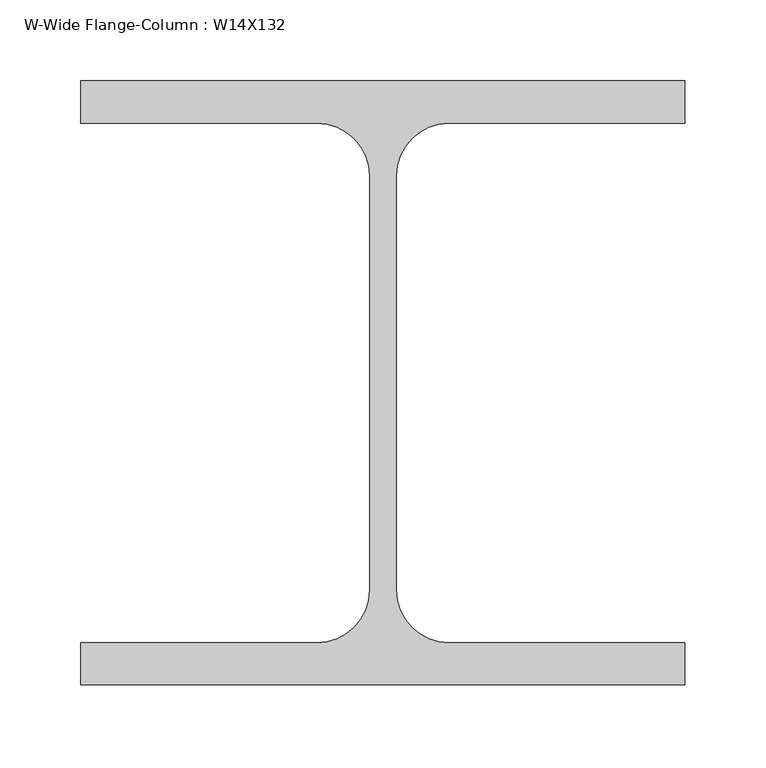
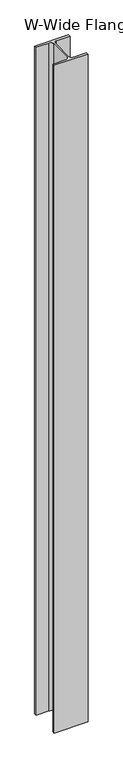
"""IFC4 building model written with IfcOpenShell, lengths in millimetres: column geometry, W-Wide Flange-Column : W14X132."""

from ifc_helpers import new_model, si_unit, point, frame, frame_2d, origin, place, context, project, spatial, polyline, circle_curve, trimmed, segment, composite_curve, outline, extrude, source, transform, mapped, element, save


def w_wide_flange_column_w14x132_97c2514c(model_context):
    return source(origin(), model_context, "Body", "SweptSolid", [
        extrude(outline(composite_curve([segment(polyline([(186.69, 186.69), (186.69, 160.528), (40.767, 160.528)]), True, "CONTINUOUS"), segment(trimmed(circle_curve(frame_2d((40.767, 127.9525)), 32.5755), [point((40.767, 160.528))], [point((8.1915, 127.9525))], True, "CARTESIAN"), True, "CONTINUOUS"), segment(polyline([(8.1915, 127.9525), (8.1915, -127.9525)]), True, "CONTINUOUS"), segment(trimmed(circle_curve(frame_2d((40.767, -127.9525)), 32.5755), [point((8.1915, -127.9525))], [point((40.767, -160.528))], True, "CARTESIAN"), True, "CONTINUOUS"), segment(polyline([(40.767, -160.528), (186.69, -160.528), (186.69, -186.69), (-186.69, -186.69), (-186.69, -160.528), (-40.767, -160.528)]), True, "CONTINUOUS"), segment(trimmed(circle_curve(frame_2d((-40.767, -127.9525)), 32.5755), [point((-40.767, -160.528))], [point((-8.1915, -127.9525))], True, "CARTESIAN"), True, "CONTINUOUS"), segment(polyline([(-8.1915, -127.9525), (-8.1915, 127.9525)]), True, "CONTINUOUS"), segment(trimmed(circle_curve(frame_2d((-40.767, 127.9525)), 32.5755), [point((-8.1915, 127.9525))], [point((-40.767, 160.528))], True, "CARTESIAN"), True, "CONTINUOUS"), segment(polyline([(-40.767, 160.528), (-186.69, 160.528), (-186.69, 186.69), (186.69, 186.69)]), True, "CONTINUOUS")], self_intersect=False)), frame((0.0, 0.0, -304.8), z_axis=(0.0, 0.0, 1.0), x_axis=(1.0, 0.0, 0.0)), (0.0, 0.0, 1.0), 7797.8),
    ])


if __name__ == "__main__":
    model = new_model("IFC4")
    model_context = context("Model", 3, world=origin())
    ifc_project = project(units=[si_unit("LENGTHUNIT", "METRE", prefix="MILLI")], contexts=[model_context])
    site = spatial("IfcSite", under=ifc_project)
    building = spatial("IfcBuilding", under=site)
    placement = place(None, origin())
    w_wide_flange_column_w14x132_shape = w_wide_flange_column_w14x132_97c2514c(model_context)
    element("IfcColumn", 1, ObjectType="W-Wide Flange-Column : W14X132", at=placement, inside=building, context=model_context, shape_type="MappedRepresentation", body=[
        mapped(w_wide_flange_column_w14x132_shape, transform((0.0, 0.0, 0.0), x_axis=(1.0, 0.0, 0.0), y_axis=(0.0, 1.0, 0.0), z_axis=(0.0, 0.0, 1.0))),
    ])
    save(model, "model.ifc")

# Revit data of these elements
# Type "W-Wide Flange-Column : W14X132"
#   Assembly Code = "B10"
#   W = 132
#   bf = 1' - 2.7"
#   d = 1' - 2.7"
#   k = 0' - 2 5/16"
#   kr = 0' - 1.2825"
#   tf = 0' - 1.03"
#   tw = 0' - 0.645"
#   A = 0.269444 SF
#   Column Material [instance default] = Metal - Steel - ASTM A992
# Element 1 (IfcColumn, "W-Wide Flange-Column : W14X132")
#   Materials on its faces: "Metal - Steel - ASTM A992"
# Materials
#   "Metal - Steel - ASTM A992": class "Metal", colour RGB 128 0 0, transparency 0
